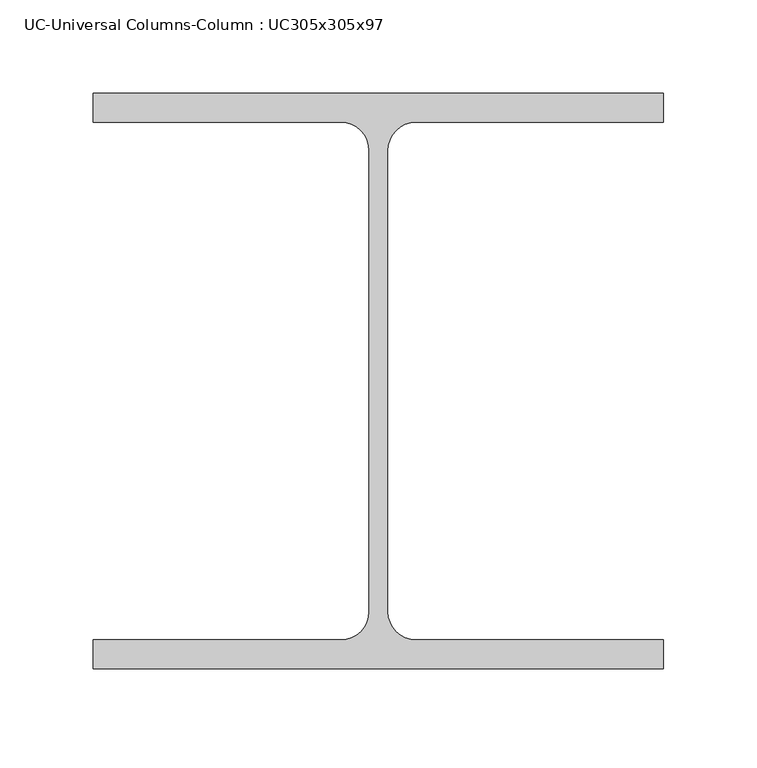
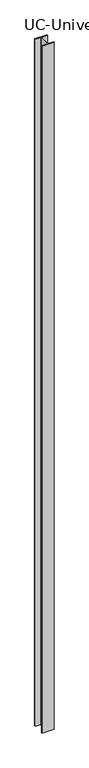
"""IFC4 building model written with IfcOpenShell, lengths in millimetres: column geometry, UC-Universal Columns-Column : UC305x305x97."""

import ifcopenshell
import ifcopenshell.guid

model = None  # the IFC model being written
_history = None  # IfcOwnerHistory: only IFC2X3 demands one
_inside = {}  # id of a spatial element -> (the spatial element, [elements in it])
_under = {}  # id of a project, library or spatial element -> (it, [spatial elements below it])
_declared = {}  # id of a project -> (the project, [libraries it declares])
_typed = {}  # id of a type object -> (the type object, [elements of that type])
_made_of = {}  # id of a material, layer set ... -> (it, [elements and type objects made of it])


def new_model(schema):
    """Start an empty IFC model of exactly this schema.

    Asked for "IFC4X3", IfcOpenShell would pick the latest addendum, in which some entities
    have other attributes; the version numbers below select the first issue.
    IFC2X3 requires an IfcOwnerHistory on every rooted entity: one is made here for all.
    """
    global model, _history
    if schema == "IFC4X3":
        model = ifcopenshell.file(schema_version=(4, 3, 0, 0))
    else:
        model = ifcopenshell.file(schema=schema)
    _inside.clear()
    _under.clear()
    _declared.clear()
    _typed.clear()
    _made_of.clear()
    _history = None
    if model.schema == "IFC2X3":
        org = make("IfcOrganization", Name="unknown")
        user = make(
            "IfcPersonAndOrganization",
            ThePerson=make("IfcPerson", FamilyName="unknown"),
            TheOrganization=org,
        )
        app = make(
            "IfcApplication",
            ApplicationDeveloper=org,
            Version="unknown",
            ApplicationFullName="unknown",
            ApplicationIdentifier="unknown",
        )
        _history = make(
            "IfcOwnerHistory",
            OwningUser=user,
            OwningApplication=app,
            ChangeAction="ADDED",
            CreationDate=0,
        )
    return model


def make(cls, **values):
    """One entity of the class cls with the attributes given. An attribute that is None is left unset."""
    return model.create_entity(
        cls, **{name: value for name, value in values.items() if value is not None}
    )


def rooted(cls, **values):
    """An entity with a GlobalId (a new one), such as an element, a storey or a relation."""
    return make(cls, GlobalId=ifcopenshell.guid.new(), OwnerHistory=_history, **values)


def si_unit(unit_type, name, prefix=None):
    """IfcSIUnit, for example si_unit("LENGTHUNIT", "METRE", prefix="MILLI")."""
    return make("IfcSIUnit", UnitType=unit_type, Prefix=prefix, Name=name)


def assignment(units):
    """IfcUnitAssignment: the units of a project."""
    return None if units is None else make("IfcUnitAssignment", Units=units)


def point(xyz):
    """IfcCartesianPoint."""
    return None if xyz is None else make("IfcCartesianPoint", Coordinates=xyz)


def direction(xyz):
    """IfcDirection."""
    return None if xyz is None else make("IfcDirection", DirectionRatios=xyz)


def frame(location, z_axis=None, x_axis=None):
    """IfcAxis2Placement3D, a coordinate frame: its origin and axes. An axis left out is left unset."""
    return make(
        "IfcAxis2Placement3D",
        Location=point(location),
        Axis=direction(z_axis),
        RefDirection=direction(x_axis),
    )


def frame_2d(location, x_axis=None):
    """IfcAxis2Placement2D, a coordinate frame in the plane: its origin and x axis."""
    return make(
        "IfcAxis2Placement2D", Location=point(location), RefDirection=direction(x_axis)
    )


def origin():
    """The frame at (0, 0, 0) with its axes left unset."""
    return frame((0.0, 0.0, 0.0))


def place(relative_to, where):
    """IfcLocalPlacement: puts the frame where relative to a parent placement (None: the world)."""
    return make(
        "IfcLocalPlacement", PlacementRelTo=relative_to, RelativePlacement=where
    )


def context(
    kind, dimensions, precision=None, world=None, true_north=None, identifier=None
):
    """IfcGeometricRepresentationContext, for example the 3D "Model" context."""
    return make(
        "IfcGeometricRepresentationContext",
        ContextIdentifier=identifier,
        ContextType=kind,
        CoordinateSpaceDimension=dimensions,
        Precision=precision,
        WorldCoordinateSystem=world,
        TrueNorth=true_north,
    )


def project(units=None, contexts=None):
    """IfcProject with its units and contexts."""
    return rooted(
        "IfcProject",
        Name="project",
        RepresentationContexts=contexts,
        UnitsInContext=assignment(units),
    )


def spatial(cls, under=None, at=None, **own):
    """A site, building, storey or space (cls), placed at a placement, below another one or the project."""
    s = rooted(cls, ObjectPlacement=at, **own)
    if under is not None:
        _under.setdefault(under.id(), (under, []))[1].append(s)
    return s


def polyline(points):
    """IfcPolyline through the points."""
    return make("IfcPolyline", Points=[point(p) for p in points])


def circle_curve(where, radius):
    """IfcCircle in the frame where."""
    return make("IfcCircle", Position=where, Radius=radius)


def trimmed(basis, trim1, trim2, sense, master):
    """IfcTrimmedCurve: the piece of a basis curve between two trims."""
    return make(
        "IfcTrimmedCurve",
        BasisCurve=basis,
        Trim1=trim1,
        Trim2=trim2,
        SenseAgreement=sense,
        MasterRepresentation=master,
    )


def segment(curve, same_sense, transition):
    """IfcCompositeCurveSegment."""
    return make(
        "IfcCompositeCurveSegment",
        Transition=transition,
        SameSense=same_sense,
        ParentCurve=curve,
    )


def composite_curve(segments, self_intersect=None):
    """IfcCompositeCurve: segments joined end to end."""
    return make("IfcCompositeCurve", Segments=segments, SelfIntersect=self_intersect)


def outline(outer, holes=None, kind="AREA"):
    """IfcArbitraryClosedProfileDef: a profile drawn as a closed curve; with holes, ...WithVoids."""
    if holes is None:
        return make("IfcArbitraryClosedProfileDef", ProfileType=kind, OuterCurve=outer)
    return make(
        "IfcArbitraryProfileDefWithVoids",
        ProfileType=kind,
        OuterCurve=outer,
        InnerCurves=holes,
    )


def extrude(swept, where, along, depth):
    """IfcExtrudedAreaSolid: the profile swept, set in the frame where, extruded along a direction by depth."""
    return make(
        "IfcExtrudedAreaSolid",
        SweptArea=swept,
        Position=where,
        ExtrudedDirection=direction(along),
        Depth=depth,
    )


def shape(context_of_items, identifier, shape_type, items):
    """IfcShapeRepresentation: the items that make up one representation, for example the "Body"."""
    return make(
        "IfcShapeRepresentation",
        ContextOfItems=context_of_items,
        RepresentationIdentifier=identifier,
        RepresentationType=shape_type,
        Items=items,
    )


def source(mapping_origin, context_of_items, identifier, shape_type, items):
    """IfcRepresentationMap: a shape defined once, which mapped items show again and again."""
    return make(
        "IfcRepresentationMap",
        MappingOrigin=mapping_origin,
        MappedRepresentation=shape(context_of_items, identifier, shape_type, items),
    )


def transform(
    local_origin,
    x_axis=None,
    y_axis=None,
    z_axis=None,
    scale=None,
    scale2=None,
    scale3=None,
    uniform=True,
):
    """IfcCartesianTransformationOperator3D, or its non-uniform kind. x_axis, y_axis, z_axis: its Axis1, 2, 3."""
    if uniform:
        return make(
            "IfcCartesianTransformationOperator3D",
            Axis1=direction(x_axis),
            Axis2=direction(y_axis),
            LocalOrigin=point(local_origin),
            Scale=scale,
            Axis3=direction(z_axis),
        )
    return make(
        "IfcCartesianTransformationOperator3DnonUniform",
        Axis1=direction(x_axis),
        Axis2=direction(y_axis),
        LocalOrigin=point(local_origin),
        Scale=scale,
        Axis3=direction(z_axis),
        Scale2=scale2,
        Scale3=scale3,
    )


def mapped(mapping_source, mapping_target):
    """IfcMappedItem: shows the shape of a source again, moved by a transform."""
    return make(
        "IfcMappedItem", MappingSource=mapping_source, MappingTarget=mapping_target
    )


def made_of(thing, what):
    """Note that an element or type object is made of a material, layer set ...; save() writes the relation."""
    if what is not None:
        _made_of.setdefault(what.id(), (what, []))[1].append(thing)
    return thing


def element(
    cls,
    number,
    at=None,
    inside=None,
    cuts=None,
    type_object=None,
    material=None,
    context=None,
    identifier="Body",
    shape_type=None,
    held_by="IfcProductDefinitionShape",
    body=None,
    shapes=None,
    **own,
):
    """One element of the class cls, such as IfcWall. Its Tag is "e" and its number.

    at: its placement. inside: the storey or other place that contains it. cuts: it is an
    opening in that element (IfcRelVoidsElement). A single representation is given by context,
    identifier, shape_type and body (its items); several are given by shapes. held_by: the class
    of the entity that holds the representations. save() writes the other relations.
    """
    e = rooted(cls, Tag="e%d" % number, ObjectPlacement=at, **own)
    if body is not None:
        shapes = [shape(context, identifier, shape_type, body)]
    if shapes is not None:
        e.Representation = make(held_by, Representations=shapes)
    if inside is not None:
        _inside.setdefault(inside.id(), (inside, []))[1].append(e)
    if cuts is not None:
        rooted(
            "IfcRelVoidsElement", RelatingBuildingElement=cuts, RelatedOpeningElement=e
        )
    if type_object is not None:
        _typed.setdefault(type_object.id(), (type_object, []))[1].append(e)
    return made_of(e, material)


def aggregate(whole, parts):
    """IfcRelAggregates: a whole, such as a stair, and the parts it consists of."""
    return rooted("IfcRelAggregates", RelatingObject=whole, RelatedObjects=parts)


def save(model, path):
    """Write the relations noted so far, then the file.

    IfcRelAggregates (storeys below a building ...), IfcRelContainedInSpatialStructure (elements
    in a storey), IfcRelDefinesByType, IfcRelAssociatesMaterial and IfcRelDeclares: one each for
    every whole, place, type object, material and project.
    """
    for whole, parts in _under.values():
        aggregate(whole, parts)
    for where, things in _inside.values():
        rooted(
            "IfcRelContainedInSpatialStructure",
            RelatedElements=things,
            RelatingStructure=where,
        )
    for kind, things in _typed.values():
        rooted("IfcRelDefinesByType", RelatedObjects=things, RelatingType=kind)
    for what, things in _made_of.values():
        rooted("IfcRelAssociatesMaterial", RelatedObjects=things, RelatingMaterial=what)
    for by, libraries in _declared.values():
        rooted("IfcRelDeclares", RelatingContext=by, RelatedDefinitions=libraries)
    model.write(path)


def uc_universal_columns_column_uc305x305x97_e2fb10fc(model_context):
    return source(origin(), model_context, "Body", "SweptSolid", [
        extrude(outline(composite_curve([segment(polyline([(152.65, 153.95), (152.65, 138.55), (20.15, 138.55)]), True, "CONTINUOUS"), segment(trimmed(circle_curve(frame_2d((20.15, 123.35)), 15.2), [point((20.15, 138.55))], [point((4.95, 123.35))], True, "CARTESIAN"), True, "CONTINUOUS"), segment(polyline([(4.95, 123.35), (4.95, -123.35)]), True, "CONTINUOUS"), segment(trimmed(circle_curve(frame_2d((20.15, -123.35)), 15.2), [point((4.95, -123.35))], [point((20.15, -138.55))], True, "CARTESIAN"), True, "CONTINUOUS"), segment(polyline([(20.15, -138.55), (152.65, -138.55), (152.65, -153.95), (-152.65, -153.95), (-152.65, -138.55), (-20.15, -138.55)]), True, "CONTINUOUS"), segment(trimmed(circle_curve(frame_2d((-20.15, -123.35)), 15.2), [point((-20.15, -138.55))], [point((-4.95, -123.35))], True, "CARTESIAN"), True, "CONTINUOUS"), segment(polyline([(-4.95, -123.35), (-4.95, 123.35)]), True, "CONTINUOUS"), segment(trimmed(circle_curve(frame_2d((-20.15, 123.35)), 15.2), [point((-4.95, 123.35))], [point((-20.15, 138.55))], True, "CARTESIAN"), True, "CONTINUOUS"), segment(polyline([(-20.15, 138.55), (-152.65, 138.55), (-152.65, 153.95), (152.65, 153.95)]), True, "CONTINUOUS")], self_intersect=False)), frame((0.0, 0.0, -5550.0), z_axis=(0.0, 0.0, 1.0), x_axis=(1.0, 0.0, 0.0)), (0.0, 0.0, 1.0), 17989.0),
    ])


if __name__ == "__main__":
    model = new_model("IFC4")
    model_context = context("Model", 3, world=origin())
    ifc_project = project(units=[si_unit("LENGTHUNIT", "METRE", prefix="MILLI")], contexts=[model_context])
    site = spatial("IfcSite", under=ifc_project)
    building = spatial("IfcBuilding", under=site)
    placement = place(None, origin())
    uc_universal_columns_column_uc305x305x97_shape = uc_universal_columns_column_uc305x305x97_e2fb10fc(model_context)
    element("IfcColumn", 1, ObjectType="UC-Universal Columns-Column : UC305x305x97", at=placement, inside=building, context=model_context, shape_type="MappedRepresentation", body=[
        mapped(uc_universal_columns_column_uc305x305x97_shape, transform((0.0, 0.0, 0.0), x_axis=(1.0, 0.0, 0.0), y_axis=(0.0, 1.0, 0.0), z_axis=(0.0, 0.0, 1.0))),
    ])
    save(model, "model.ifc")

# Revit data of these elements
# Type "UC-Universal Columns-Column : UC305x305x97"
#   Section Name Key = "UC305x305x97"
#   Cost = 2
#   Width = 30.53 cm
#   Web Thickness = 0.99 cm
#   Web Fillet = 1.52 cm
#   Warping Constant = 1560000.0 cm⁶
#   Torsional Moment of Inertia = 91.20 cm⁴
#   Section Area = 123.0 cm²
#   Plastic Modulus weak axis = 726.0 cm³
#   Plastic Modulus strong axis = 1592.0 cm³
#   Nominal Weight = 96.8996 kgf/m
#   Moment of Inertia weak axis = 7308.00 cm⁴
#   Moment of Inertia strong axis = 22249.00 cm⁴
#   Height = 30.79 cm
#   Flange Thickness = 1.54 cm
#   Elastic Modulus weak axis = 479.0 cm³
#   Elastic Modulus strong axis = 1445.0 cm³
#   Centroid Vertical = 15.395 cm
#   Centroid Horizontal = 15.265 cm
#   Bolt Spacing = 14.0 cm
#   Structural Material [instance default] = Metal - Steel 43-275
#   Type Comments = ""
#   Assembly Code = ""
# Element 1 (IfcColumn, "UC-Universal Columns-Column : UC305x305x97")
#   Materials on its faces: "Metal - Steel 43-275"
# Materials
#   "Metal - Steel 43-275": class "Metal", colour RGB 247 247 247, transparency 0, Cost = 0
